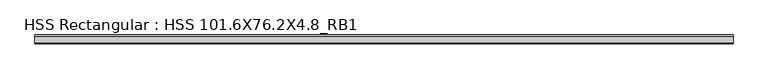
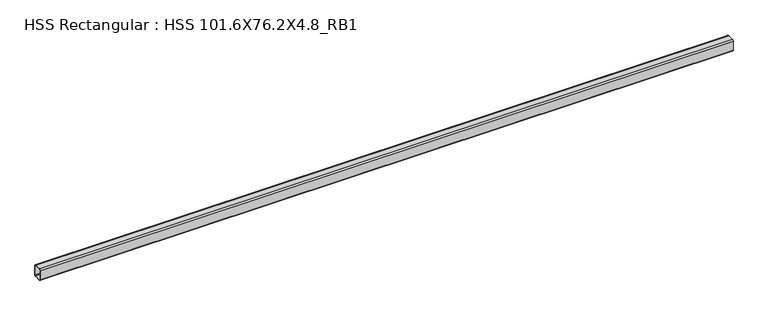
"""IFC4 building model written with IfcOpenShell, lengths in millimetres: beam geometry, HSS Rectangular : HSS 101.6X76.2X4.8_RB1."""

from ifc_helpers import new_model, si_unit, point, frame, frame_2d, origin, place, context, project, spatial, polyline, circle_curve, trimmed, segment, composite_curve, outline, extrude, source, transform, mapped, element, save


def hss_rectangular_hss_101_6x76_2x4_8_rb1_9e273c7a(model_context):
    return source(origin(), model_context, "Body", "SweptSolid", [
        extrude(outline(composite_curve([segment(polyline([(38.1, 41.275), (38.1, -41.275)]), True, "CONTINUOUS"), segment(trimmed(circle_curve(frame_2d((28.575, -41.275)), 9.525), [point((38.1, -41.275))], [point((28.575, -50.8))], False, "CARTESIAN"), True, "CONTINUOUS"), segment(polyline([(28.575, -50.8), (-28.575, -50.8)]), True, "CONTINUOUS"), segment(trimmed(circle_curve(frame_2d((-28.575, -41.275)), 9.525), [point((-28.575, -50.8))], [point((-38.1, -41.275))], False, "CARTESIAN"), True, "CONTINUOUS"), segment(polyline([(-38.1, -41.275), (-38.1, 41.275)]), True, "CONTINUOUS"), segment(trimmed(circle_curve(frame_2d((-28.575, 41.275)), 9.525), [point((-38.1, 41.275))], [point((-28.575, 50.8))], False, "CARTESIAN"), True, "CONTINUOUS"), segment(polyline([(-28.575, 50.8), (28.575, 50.8)]), True, "CONTINUOUS"), segment(trimmed(circle_curve(frame_2d((28.575, 41.275)), 9.525), [point((28.575, 50.8))], [point((38.1, 41.275))], False, "CARTESIAN"), True, "CONTINUOUS")], self_intersect=False), holes=[composite_curve([segment(trimmed(circle_curve(frame_2d((-28.575, 41.275)), 4.7625), [point((-28.575, 46.0375))], [point((-33.3375, 41.275))], True, "CARTESIAN"), True, "CONTINUOUS"), segment(polyline([(-33.3375, 41.275), (-33.3375, -41.275)]), True, "CONTINUOUS"), segment(trimmed(circle_curve(frame_2d((-28.575, -41.275)), 4.7625), [point((-33.3375, -41.275))], [point((-28.575, -46.0375))], True, "CARTESIAN"), True, "CONTINUOUS"), segment(polyline([(-28.575, -46.0375), (28.575, -46.0375)]), True, "CONTINUOUS"), segment(trimmed(circle_curve(frame_2d((28.575, -41.275)), 4.7625), [point((28.575, -46.0375))], [point((33.3375, -41.275))], True, "CARTESIAN"), True, "CONTINUOUS"), segment(polyline([(33.3375, -41.275), (33.3375, 41.275)]), True, "CONTINUOUS"), segment(trimmed(circle_curve(frame_2d((28.575, 41.275)), 4.7625), [point((33.3375, 41.275))], [point((28.575, 46.0375))], True, "CARTESIAN"), True, "CONTINUOUS"), segment(polyline([(28.575, 46.0375), (-28.575, 46.0375)]), True, "CONTINUOUS")], self_intersect=False)]), frame((1645.6863857, 0.0, 0.0), z_axis=(1.0, 0.0, 0.0), x_axis=(0.0, 1.0, 0.0)), (0.0, 0.0, 1.0), 5913.5382104),
    ])


if __name__ == "__main__":
    model = new_model("IFC4")
    model_context = context("Model", 3, world=origin())
    ifc_project = project(units=[si_unit("LENGTHUNIT", "METRE", prefix="MILLI")], contexts=[model_context])
    site = spatial("IfcSite", under=ifc_project)
    building = spatial("IfcBuilding", under=site)
    placement = place(None, origin())
    hss_rectangular_hss_101_6x76_2x4_8_rb1_shape = hss_rectangular_hss_101_6x76_2x4_8_rb1_9e273c7a(model_context)
    element("IfcBeam", 1, ObjectType="HSS Rectangular : HSS 101.6X76.2X4.8_RB1", at=placement, inside=building, context=model_context, shape_type="MappedRepresentation", body=[
        mapped(hss_rectangular_hss_101_6x76_2x4_8_rb1_shape, transform((0.0, 0.0, 0.0), x_axis=(1.0, 0.0, 0.0), y_axis=(0.0, 1.0, 0.0), z_axis=(0.0, 0.0, 1.0))),
    ])
    save(model, "model.ifc")

# Revit data of these elements
# Type "HSS Rectangular : HSS 101.6X76.2X4.8_RB1"
#   Section Name Key = "HSS 4X3X3/16"
#   Assembly Code = "B10"
#   Width = 7.62 cm
#   Wall Nominal Thickness = 0.4763 cm
#   Wall Design Thickness = 0.442 cm
#   Torsional Moment of Inertia = 260.561 cm⁴
#   Torsional Modulus = 61.2876 cm³
#   Section Area = 14.4516 cm²
#   Plastic Modulus weak axis = 40.3122 cm³
#   Plastic Modulus strong axis = 49.1612 cm³
#   Perimeter = 0.881482 m²/m
#   Outer Fillet = 0.9525 cm
#   Nominal Weight = 12.1285 kgf/m
#   Moment of Inertia weak axis = 131.529 cm⁴
#   Moment of Inertia strong axis = 205.202 cm⁴
#   Inner Fillet = 0.4763 cm
#   Height = 10.16 cm
#   Elastic Modulus weak axis = 34.4128 cm³
#   Elastic Modulus strong axis = 40.476 cm³
#   Centroid Vertical = 5.08 cm
#   Centroid Horizontal = 3.81 cm
#   Length [instance default] = 1524 mm
#   Structural Material [instance default] = Steel ASTM A500, Grade B, Rectangular and Square
#   Principal Axes Angle = 0
# Element 1 (IfcBeam, "HSS Rectangular : HSS 101.6X76.2X4.8_RB1")
#   Structural Material = Steel ASTM A992
#   Materials on its faces: "Steel ASTM A992"
# Materials
#   "Steel ASTM A500, Grade B, Rectangular and Square": class "Metal", colour RGB 199 199 199, transparency 0, Description = "Carbon steel", Cost = 0
#   "Steel ASTM A992": class "Metal", colour RGB 199 199 199, transparency 0, Description = "Structural steel 50ksi", Cost = 0
